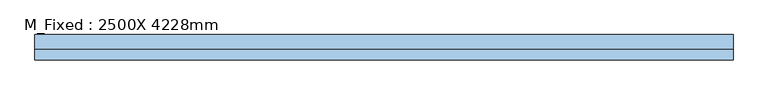
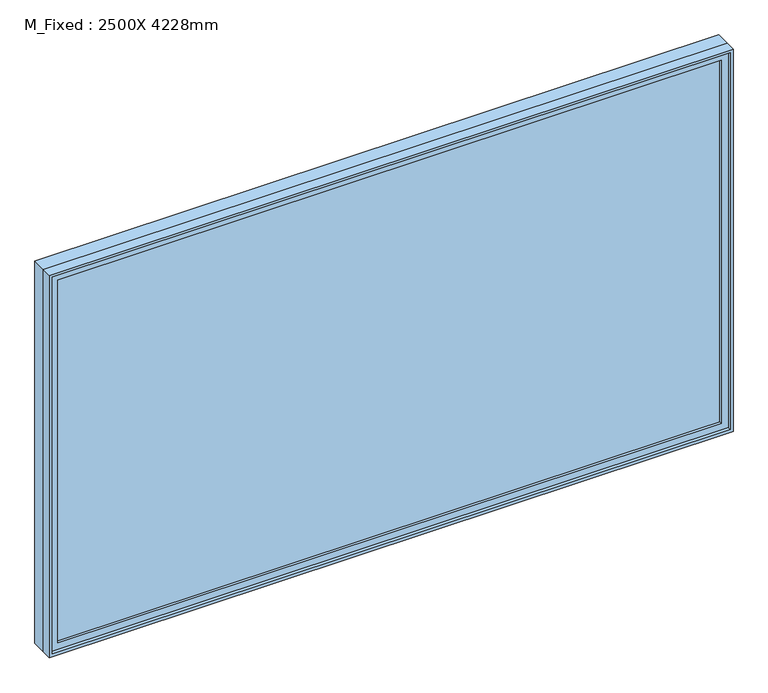
"""IFC4 building model written with IfcOpenShell, lengths in millimetres: window geometry, M_Fixed : 2500X 4228mm."""

from ifc_helpers import new_model, si_unit, frame, origin, place, context, project, spatial, polyline, outline, extrude, source, transform, mapped, element, save


def m_fixed_2500x_4228mm_f14c179f(model_context):
    return source(origin(), model_context, "Body", "SweptSolid", [
        extrude(outline(polyline([(-2050.8, -54.2), (-2050.8, -42.2), (2050.8, -42.2), (2050.8, -54.2), (-2050.8, -54.2)])), frame((0.0, 0.0, 368.0), z_axis=(0.0, 0.0, 1.0), x_axis=(1.0, 0.0, 0.0)), (0.0, 0.0, 1.0), 2374.0),
        extrude(outline(polyline([(2786.0, -2094.8), (324.0, -2094.8), (324.0, 2094.8), (2786.0, 2094.8), (2786.0, -2094.8)]), holes=[polyline([(2742.0, -2050.8), (2742.0, 2050.8), (368.0, 2050.8), (368.0, -2050.8), (2742.0, -2050.8)])]), frame((0.0, -70.2, 0.0), z_axis=(0.0, 1.0, 0.0), x_axis=(0.0, 0.0, 1.0)), (0.0, 0.0, 1.0), 44.0),
        extrude(outline(polyline([(2805.0, -2113.8), (305.0, -2113.8), (305.0, 2113.8), (2805.0, 2113.8), (2805.0, -2113.8)]), holes=[polyline([(2786.0, -2094.8), (2786.0, 2094.8), (324.0, 2094.8), (324.0, -2094.8), (2786.0, -2094.8)])]), frame((0.0, -89.2, 0.0), z_axis=(0.0, 1.0, 0.0), x_axis=(0.0, 0.0, 1.0)), (0.0, 0.0, 1.0), 63.0),
        extrude(outline(polyline([(2805.0, -2113.8), (305.0, -2113.8), (305.0, 2113.8), (2805.0, 2113.8), (2805.0, -2113.8)]), holes=[polyline([(2773.0, -2081.8), (2773.0, 2081.8), (337.0, 2081.8), (337.0, -2081.8), (2773.0, -2081.8)])]), frame((0.0, -26.2, 0.0), z_axis=(0.0, 1.0, 0.0), x_axis=(0.0, 0.0, 1.0)), (0.0, 0.0, 1.0), 89.4),
    ])


if __name__ == "__main__":
    model = new_model("IFC4")
    model_context = context("Model", 3, world=origin())
    ifc_project = project(units=[si_unit("LENGTHUNIT", "METRE", prefix="MILLI")], contexts=[model_context])
    site = spatial("IfcSite", under=ifc_project)
    building = spatial("IfcBuilding", under=site)
    placement = place(None, origin())
    m_fixed_2500x_4228mm_shape = m_fixed_2500x_4228mm_f14c179f(model_context)
    element("IfcWindow", 1, ObjectType="M_Fixed : 2500X 4228mm", at=placement, inside=building, context=model_context, shape_type="MappedRepresentation", body=[
        mapped(m_fixed_2500x_4228mm_shape, transform((0.0, 0.0, 0.0), x_axis=(1.0, 0.0, 0.0), y_axis=(0.0, 1.0, 0.0), z_axis=(0.0, 0.0, 1.0))),
    ])
    save(model, "model.ifc")

# Revit data of these elements
# Type "M_Fixed : 2500X 4228mm"
#   Type Mark = "25"
#   Height = 2500 mm
#   Default Sill Height = 305 mm
#   Width = 4227.6 mm
#   Window Inset = 19 mm
#   Frame Exterior Material = Sash
#   Frame Interior Material = Sash
#   Glass Pane Material = Glass
#   Sash = Sash
#   Wall Closure = (empty or 0)
# Element 1 (IfcWindow, "M_Fixed : 2500X 4228mm")
#   Materials on its faces: "Sash", "Glass"
# Materials
#   "Sash": class "Wood", colour RGB 136 99 55, transparency 0
#   "Glass": class "Glass", colour RGB 0 128 192, transparency 0.9, Description = "Soda Lime Glass", Cost = 0
